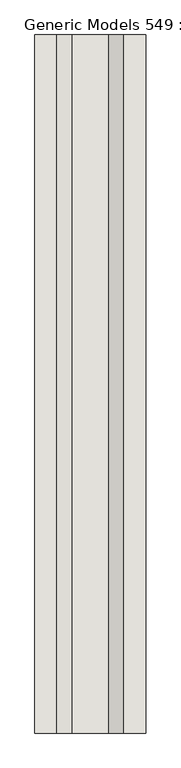
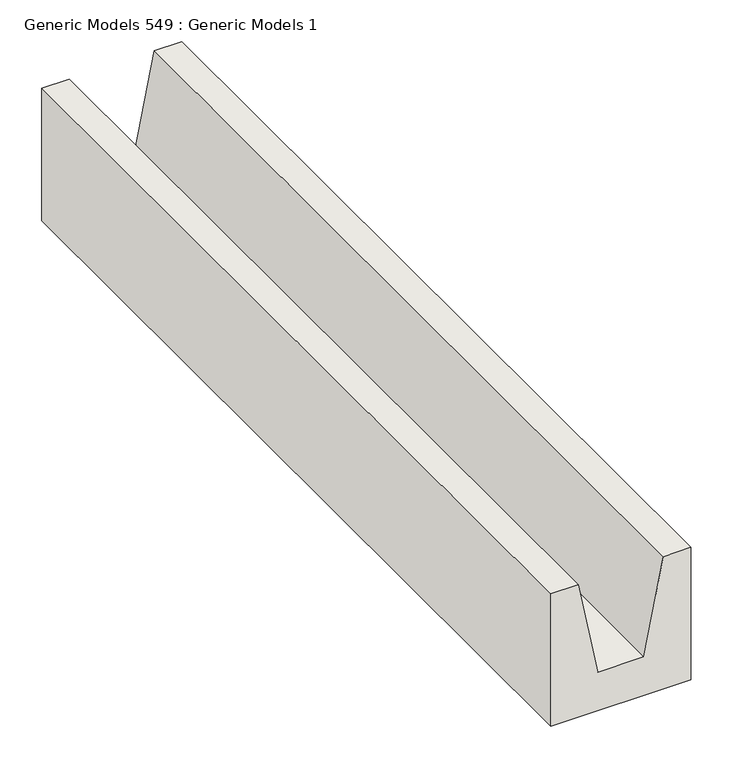
"""IFC4 building model written with IfcOpenShell, lengths in millimetres: wall geometry, Generic Models 549 : Generic Models 1."""

from ifc_helpers import new_model, si_unit, frame, origin, place, context, project, spatial, polyline, outline, extrude, source, transform, mapped, element, save


def generic_models_549_generic_models_1_e0daab97(model_context):
    return source(origin(), model_context, "Body", "SweptSolid", [
        extrude(outline(polyline([(1838.325, 148369.3375), (1838.325, 148563.0125), (2032.0, 148563.0125), (2032.0, 148524.9125), (1894.8666825, 148498.2564833), (1894.8666825, 148434.0935167), (2032.0, 148407.4375), (2032.0, 148369.3375), (1838.325, 148369.3375)])), frame((0.0, 0.0, 0.0), z_axis=(0.0, 1.0, 0.0), x_axis=(0.0, 0.0, 1.0)), (0.0, 0.0, 1.0), 1219.2),
    ])


if __name__ == "__main__":
    model = new_model("IFC4")
    model_context = context("Model", 3, world=origin())
    ifc_project = project(units=[si_unit("LENGTHUNIT", "METRE", prefix="MILLI")], contexts=[model_context])
    site = spatial("IfcSite", under=ifc_project)
    building = spatial("IfcBuilding", under=site)
    placement = place(None, origin())
    generic_models_549_generic_models_1_shape = generic_models_549_generic_models_1_e0daab97(model_context)
    element("IfcWall", 1, ObjectType="Generic Models 549 : Generic Models 1", at=placement, inside=building, context=model_context, shape_type="MappedRepresentation", body=[
        mapped(generic_models_549_generic_models_1_shape, transform((0.0, 0.0, 0.0), x_axis=(1.0, 0.0, 0.0), y_axis=(0.0, 1.0, 0.0), z_axis=(0.0, 0.0, 1.0))),
    ])
    save(model, "model.ifc")

# Revit data of these elements
# Element 1 (IfcWall, "Generic Models 549 : Generic Models 1")
#   Materials on its faces: "BOND BEAM W/ (1) CONT. #5 BAR CONT."
# Materials
#   "BOND BEAM W/ (1) CONT. #5 BAR CONT.": class "Masonry", colour RGB 203 203 199, transparency 0, Description = "Concrete masonry units", Cost = 0
